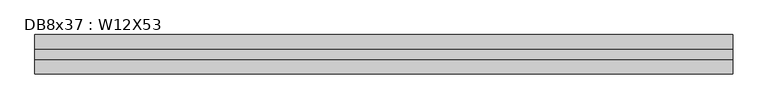
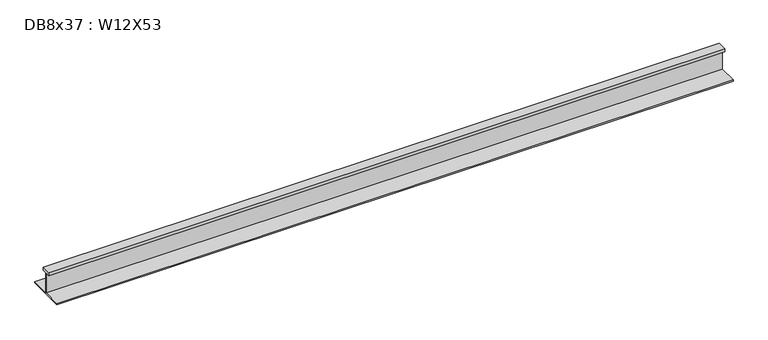
"""IFC4 building model written with IfcOpenShell, lengths in millimetres: beam geometry, DB8x37 : W12X53."""

from ifc_helpers import new_model, si_unit, frame, origin, place, context, project, spatial, polyline, outline, extrude, source, transform, mapped, element, save


def db8x37_w12x53_1efdd366(model_context):
    return source(origin(), model_context, "Body", "SweptSolid", [
        extrude(outline(polyline([(38.1, 145.415), (38.1, 120.015), (2.921, 120.015), (2.921, -48.4505), (152.4, -48.4505), (152.4, -58.1025), (-152.4, -58.1025), (-152.4, -48.4505), (-2.921, -48.4505), (-2.921, 120.015), (-38.1, 120.015), (-38.1, 145.415), (38.1, 145.415)])), frame((-2708.529, 0.0, 0.0), z_axis=(1.0, 0.0, 0.0), x_axis=(0.0, 1.0, 0.0)), (0.0, 0.0, 1.0), 5386.959),
    ])


if __name__ == "__main__":
    model = new_model("IFC4")
    model_context = context("Model", 3, world=origin())
    ifc_project = project(units=[si_unit("LENGTHUNIT", "METRE", prefix="MILLI")], contexts=[model_context])
    site = spatial("IfcSite", under=ifc_project)
    building = spatial("IfcBuilding", under=site)
    placement = place(None, origin())
    db8x37_w12x53_shape = db8x37_w12x53_1efdd366(model_context)
    element("IfcBeam", 1, ObjectType="DB8x37 : W12X53", at=placement, inside=building, context=model_context, shape_type="MappedRepresentation", body=[
        mapped(db8x37_w12x53_shape, transform((0.0, 0.0, 0.0), x_axis=(1.0, 0.0, 0.0), y_axis=(0.0, 1.0, 0.0), z_axis=(0.0, 0.0, 1.0))),
    ])
    save(model, "model.ifc")

# Revit data of these elements
# Type "DB8x37 : W12X53"
#   Assembly Code = "B10"
#   W = 53
#   Length [instance default] = 5' - 0"
#   bf = 0' - 10"
#   d = 1' - 0.1"
#   k = 0' - 1 3/8"
#   k2 = 0' - 0.8"
#   tf = 0' - 0.575"
#   tw = 0' - 0.345"
#   A = 0.108333 SF
#   Structural Material [instance default] = Steel ASTM A992
# Element 1 (IfcBeam, "DB8x37 : W12X53")
#   Materials on its faces: "Steel ASTM A992"
# Materials
#   "Steel ASTM A992": class "Metal", colour RGB 199 199 199, transparency 0, Description = "Structural steel 50ksi", Cost = 0
